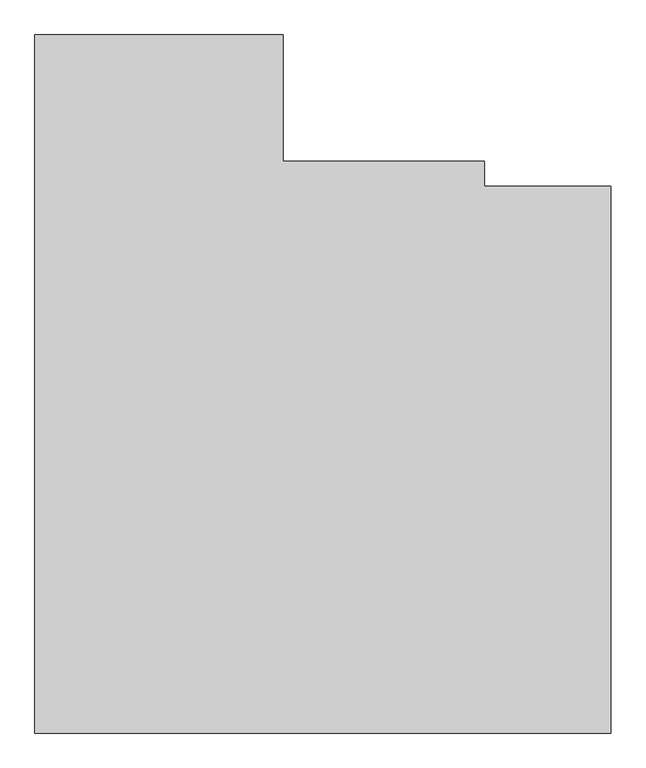
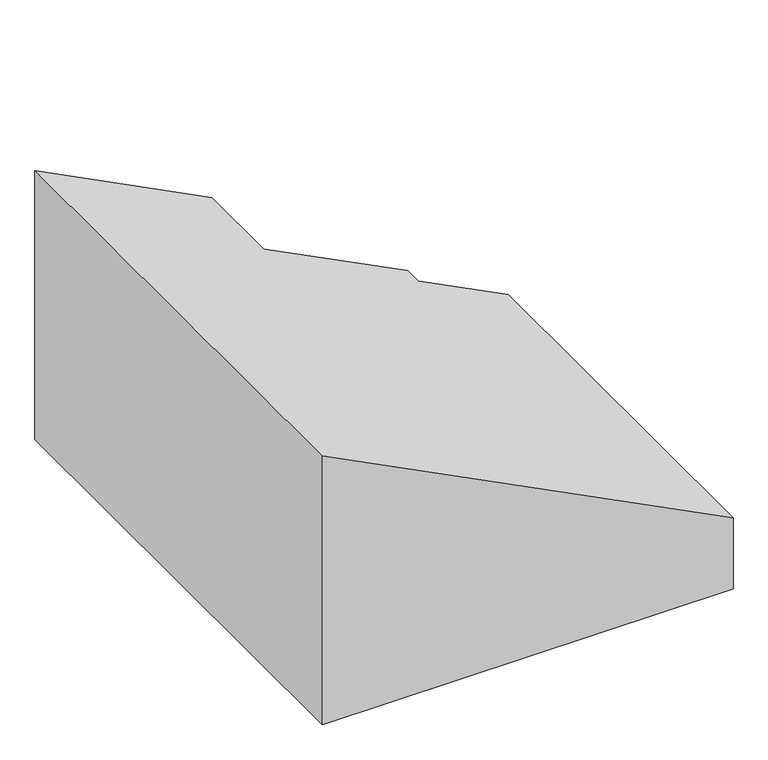
"""IFC4 building model written with IfcOpenShell, lengths in millimetres: proxy geometry, 0_3d_modell."""

import ifcopenshell
import ifcopenshell.guid

model = None  # the IFC model being written
_history = None  # IfcOwnerHistory: only IFC2X3 demands one
_inside = {}  # id of a spatial element -> (the spatial element, [elements in it])
_under = {}  # id of a project, library or spatial element -> (it, [spatial elements below it])
_declared = {}  # id of a project -> (the project, [libraries it declares])
_typed = {}  # id of a type object -> (the type object, [elements of that type])
_made_of = {}  # id of a material, layer set ... -> (it, [elements and type objects made of it])


def new_model(schema):
    """Start an empty IFC model of exactly this schema.

    Asked for "IFC4X3", IfcOpenShell would pick the latest addendum, in which some entities
    have other attributes; the version numbers below select the first issue.
    IFC2X3 requires an IfcOwnerHistory on every rooted entity: one is made here for all.
    """
    global model, _history
    if schema == "IFC4X3":
        model = ifcopenshell.file(schema_version=(4, 3, 0, 0))
    else:
        model = ifcopenshell.file(schema=schema)
    _inside.clear()
    _under.clear()
    _declared.clear()
    _typed.clear()
    _made_of.clear()
    _history = None
    if model.schema == "IFC2X3":
        org = make("IfcOrganization", Name="unknown")
        user = make(
            "IfcPersonAndOrganization",
            ThePerson=make("IfcPerson", FamilyName="unknown"),
            TheOrganization=org,
        )
        app = make(
            "IfcApplication",
            ApplicationDeveloper=org,
            Version="unknown",
            ApplicationFullName="unknown",
            ApplicationIdentifier="unknown",
        )
        _history = make(
            "IfcOwnerHistory",
            OwningUser=user,
            OwningApplication=app,
            ChangeAction="ADDED",
            CreationDate=0,
        )
    return model


def make(cls, **values):
    """One entity of the class cls with the attributes given. An attribute that is None is left unset."""
    return model.create_entity(
        cls, **{name: value for name, value in values.items() if value is not None}
    )


def rooted(cls, **values):
    """An entity with a GlobalId (a new one), such as an element, a storey or a relation."""
    return make(cls, GlobalId=ifcopenshell.guid.new(), OwnerHistory=_history, **values)


def si_unit(unit_type, name, prefix=None):
    """IfcSIUnit, for example si_unit("LENGTHUNIT", "METRE", prefix="MILLI")."""
    return make("IfcSIUnit", UnitType=unit_type, Prefix=prefix, Name=name)


def assignment(units):
    """IfcUnitAssignment: the units of a project."""
    return None if units is None else make("IfcUnitAssignment", Units=units)


def point(xyz):
    """IfcCartesianPoint."""
    return None if xyz is None else make("IfcCartesianPoint", Coordinates=xyz)


def direction(xyz):
    """IfcDirection."""
    return None if xyz is None else make("IfcDirection", DirectionRatios=xyz)


def frame(location, z_axis=None, x_axis=None):
    """IfcAxis2Placement3D, a coordinate frame: its origin and axes. An axis left out is left unset."""
    return make(
        "IfcAxis2Placement3D",
        Location=point(location),
        Axis=direction(z_axis),
        RefDirection=direction(x_axis),
    )


def origin():
    """The frame at (0, 0, 0) with its axes left unset."""
    return frame((0.0, 0.0, 0.0))


def place(relative_to, where):
    """IfcLocalPlacement: puts the frame where relative to a parent placement (None: the world)."""
    return make(
        "IfcLocalPlacement", PlacementRelTo=relative_to, RelativePlacement=where
    )


def context(
    kind, dimensions, precision=None, world=None, true_north=None, identifier=None
):
    """IfcGeometricRepresentationContext, for example the 3D "Model" context."""
    return make(
        "IfcGeometricRepresentationContext",
        ContextIdentifier=identifier,
        ContextType=kind,
        CoordinateSpaceDimension=dimensions,
        Precision=precision,
        WorldCoordinateSystem=world,
        TrueNorth=true_north,
    )


def project(units=None, contexts=None):
    """IfcProject with its units and contexts."""
    return rooted(
        "IfcProject",
        Name="project",
        RepresentationContexts=contexts,
        UnitsInContext=assignment(units),
    )


def spatial(cls, under=None, at=None, **own):
    """A site, building, storey or space (cls), placed at a placement, below another one or the project."""
    s = rooted(cls, ObjectPlacement=at, **own)
    if under is not None:
        _under.setdefault(under.id(), (under, []))[1].append(s)
    return s


def faces_of(points, faces, orient=None, outer=None):
    """IfcFace entities. A face is a list of loops; a loop is a list of indices into points, from 0.

    orient and outer hold one flag for each loop. By default every Orientation is true, the
    first loop of a face is its IfcFaceOuterBound and the others are IfcFaceBound.
    """
    made = []
    for i, loops in enumerate(faces):
        bounds = []
        for j, loop in enumerate(loops):
            is_outer = j == 0 if outer is None else outer[i][j]
            bounds.append(
                make(
                    "IfcFaceOuterBound" if is_outer else "IfcFaceBound",
                    Bound=make("IfcPolyLoop", Polygon=[points[k] for k in loop]),
                    Orientation=True if orient is None else orient[i][j],
                )
            )
        made.append(make("IfcFace", Bounds=bounds))
    return made


def faceted_brep(points, faces, orient=None, outer=None, voids=None):
    """IfcFacetedBrep: a solid bounded by flat faces; with voids (closed shells), ...WithVoids."""
    shared = [point(p) for p in points]
    hull = make("IfcClosedShell", CfsFaces=faces_of(shared, faces, orient, outer))
    if voids is None:
        return make("IfcFacetedBrep", Outer=hull)
    return make(
        "IfcFacetedBrepWithVoids",
        Outer=hull,
        Voids=[
            make(cls, CfsFaces=faces_of(shared, fs, o, b)) for cls, fs, o, b in voids
        ],
    )


def shape(context_of_items, identifier, shape_type, items):
    """IfcShapeRepresentation: the items that make up one representation, for example the "Body"."""
    return make(
        "IfcShapeRepresentation",
        ContextOfItems=context_of_items,
        RepresentationIdentifier=identifier,
        RepresentationType=shape_type,
        Items=items,
    )


def source(mapping_origin, context_of_items, identifier, shape_type, items):
    """IfcRepresentationMap: a shape defined once, which mapped items show again and again."""
    return make(
        "IfcRepresentationMap",
        MappingOrigin=mapping_origin,
        MappedRepresentation=shape(context_of_items, identifier, shape_type, items),
    )


def transform(
    local_origin,
    x_axis=None,
    y_axis=None,
    z_axis=None,
    scale=None,
    scale2=None,
    scale3=None,
    uniform=True,
):
    """IfcCartesianTransformationOperator3D, or its non-uniform kind. x_axis, y_axis, z_axis: its Axis1, 2, 3."""
    if uniform:
        return make(
            "IfcCartesianTransformationOperator3D",
            Axis1=direction(x_axis),
            Axis2=direction(y_axis),
            LocalOrigin=point(local_origin),
            Scale=scale,
            Axis3=direction(z_axis),
        )
    return make(
        "IfcCartesianTransformationOperator3DnonUniform",
        Axis1=direction(x_axis),
        Axis2=direction(y_axis),
        LocalOrigin=point(local_origin),
        Scale=scale,
        Axis3=direction(z_axis),
        Scale2=scale2,
        Scale3=scale3,
    )


def mapped(mapping_source, mapping_target):
    """IfcMappedItem: shows the shape of a source again, moved by a transform."""
    return make(
        "IfcMappedItem", MappingSource=mapping_source, MappingTarget=mapping_target
    )


def made_of(thing, what):
    """Note that an element or type object is made of a material, layer set ...; save() writes the relation."""
    if what is not None:
        _made_of.setdefault(what.id(), (what, []))[1].append(thing)
    return thing


def element(
    cls,
    number,
    at=None,
    inside=None,
    cuts=None,
    type_object=None,
    material=None,
    context=None,
    identifier="Body",
    shape_type=None,
    held_by="IfcProductDefinitionShape",
    body=None,
    shapes=None,
    **own,
):
    """One element of the class cls, such as IfcWall. Its Tag is "e" and its number.

    at: its placement. inside: the storey or other place that contains it. cuts: it is an
    opening in that element (IfcRelVoidsElement). A single representation is given by context,
    identifier, shape_type and body (its items); several are given by shapes. held_by: the class
    of the entity that holds the representations. save() writes the other relations.
    """
    e = rooted(cls, Tag="e%d" % number, ObjectPlacement=at, **own)
    if body is not None:
        shapes = [shape(context, identifier, shape_type, body)]
    if shapes is not None:
        e.Representation = make(held_by, Representations=shapes)
    if inside is not None:
        _inside.setdefault(inside.id(), (inside, []))[1].append(e)
    if cuts is not None:
        rooted(
            "IfcRelVoidsElement", RelatingBuildingElement=cuts, RelatedOpeningElement=e
        )
    if type_object is not None:
        _typed.setdefault(type_object.id(), (type_object, []))[1].append(e)
    return made_of(e, material)


def aggregate(whole, parts):
    """IfcRelAggregates: a whole, such as a stair, and the parts it consists of."""
    return rooted("IfcRelAggregates", RelatingObject=whole, RelatedObjects=parts)


def save(model, path):
    """Write the relations noted so far, then the file.

    IfcRelAggregates (storeys below a building ...), IfcRelContainedInSpatialStructure (elements
    in a storey), IfcRelDefinesByType, IfcRelAssociatesMaterial and IfcRelDeclares: one each for
    every whole, place, type object, material and project.
    """
    for whole, parts in _under.values():
        aggregate(whole, parts)
    for where, things in _inside.values():
        rooted(
            "IfcRelContainedInSpatialStructure",
            RelatedElements=things,
            RelatingStructure=where,
        )
    for kind, things in _typed.values():
        rooted("IfcRelDefinesByType", RelatedObjects=things, RelatingType=kind)
    for what, things in _made_of.values():
        rooted("IfcRelAssociatesMaterial", RelatedObjects=things, RelatingMaterial=what)
    for by, libraries in _declared.values():
        rooted("IfcRelDeclares", RelatingContext=by, RelatedDefinitions=libraries)
    model.write(path)


def generic_models_0269b9af(model_context):
    return source(origin(), model_context, "Body", "Brep", [
        faceted_brep([(4680.0, 4440.2642941, 853.3339073), (3655.0, 4440.2642941, 1375.5974931), (3655.0, 4645.0, 1375.5974931), (2015.3981634, 4645.0, 2211.0163558), (2015.0, 5670.0, 2211.2192302), (0.0, 5670.0, 3237.913011), (0.0, 0.0, 3237.913011), (4680.0, 0.0, 853.3339073), (2015.0, 5670.0, 0.0), (0.0, 5670.0, 0.0), (2015.3981634, 4645.0, 0.0), (3655.0, 4645.0, 0.0), (3655.0, 4440.2642941, 0.0), (4680.0, 4440.2642941, 0.0), (4680.0, 0.0, 0.0), (0.0, 0.0, 0.0)], [[[0, 1, 2, 3, 4, 5, 6, 7]], [[5, 4, 8, 9]], [[4, 3, 10, 8]], [[3, 2, 11, 10]], [[2, 1, 12, 11]], [[1, 0, 13, 12]], [[0, 7, 14, 13]], [[7, 6, 15, 14]], [[9, 15, 6, 5]], [[11, 12, 13, 14, 15, 9, 8, 10]]]),
    ])


if __name__ == "__main__":
    model = new_model("IFC4")
    model_context = context("Model", 3, world=origin())
    ifc_project = project(units=[si_unit("LENGTHUNIT", "METRE", prefix="MILLI")], contexts=[model_context])
    site = spatial("IfcSite", under=ifc_project)
    building = spatial("IfcBuilding", under=site)
    placement = place(None, origin())
    generic_models_shape = generic_models_0269b9af(model_context)
    element("IfcBuildingElementProxy", 1, Name="0_3d_modell", ObjectType="0_3d_modell", at=placement, inside=building, context=model_context, shape_type="MappedRepresentation", body=[
        mapped(generic_models_shape, transform((0.0, 0.0, 0.0), x_axis=(1.0, 0.0, 0.0), y_axis=(0.0, 1.0, 0.0), z_axis=(0.0, 0.0, 1.0))),
    ])
    save(model, "model.ifc")

# Revit data of these elements
# Project information
#   Organization Name = "Organization Name"
#   Organization Description = "Organization Description"
#   Building Name = "Building Name"
#   IfcOrganization = "KURIARCHITEKTEN"
#   IfcApplicationVersion = "2024.1"
#   IfcApplicationName = "Allplan"
#   IfcSite GUID = "3xMs$kp1n46ejeur8tozco"
#   IfcBuilding GUID = "0i8UyhEYT3nv9HLlo1H2X7"
#   IfcProject GUID = "2x1YFttxr4OvBiL8xtaqeA"
#   IfcDecomposes = "BVH Tammik Wohnhaus Waldrain"
#   IfcDecomposesGUID = "2x1YFttxr4OvBiL8xtaqeA"
#   IfcPropertySetList = "\"AllplanAttributes\""
#   BuildingName = "WALDRAIN"
#   SiteName = "BAUANTRAG"
#   IfcProject Name = "BVH Tammik Wohnhaus Waldrain"
#   AllplanAttributes.Land = "IFC - Land"
#   AllplanAttributes.Bundesland = "IFC - Bundesland"
#   AllplanAttributes.Prüfer = "Prüfstatiker"
#   AllplanAttributes.Bauherr = "Jeremy Tammik"
#   AllplanAttributes.Bruttogeschossfläche = "IFC - Bruttogeschossfläche"
#   AllplanAttributes.Projektleiter = "Projektleitername"
#   AllplanAttributes.Architekt = "Architektenname"
#   AllplanAttributes.Statik = "Statiker"
#   AllplanAttributes.Elektro = "Elektroplaner"
#   AllplanAttributes.Heizung = "Heizungsplaner"
#   AllplanAttributes.Sanitär = "Sanitärplaner"
#   AllplanAttributes.Bebaubare Fläche = "IFC - bebaubare Fläche"
#   AllplanAttributes.Maximale Gebäudehöhe = "IFC - Maximale Gebäudehöhe"
#   AllplanAttributes.Bruttogrundstücksfläche = "IFC - Bruttogrundstücksfläche"
#   AllplanAttributes.Normalhöhennull = "IFC - Höhe über NN"
#   AllplanAttributes.Projektvorlage = "IBD 2023"
#   AllplanAttributes.Bauvorhaben = "BVH Waldrain"
#   AllplanAttributes.Bauherr Straße = "Hühnerbergweg 30"
#   AllplanAttributes.Bauherr Plz/Ort = "79539 Lörrach"
#   AllplanAttributes.Architekt Straße = "Architektenstrasse 111"
#   AllplanAttributes.Architekt Plz/Ort = "72108 Architektenort"
#   AllplanAttributes.Bauvorhaben Straße = "Sonnenweg 6"
#   AllplanAttributes.Bauvorhaben Plz/Ort = "79539 Lörrach"
#   AllplanAttributes.Projektnummer = "2023"
#   AllplanAttributes.Architekt Telefonnummer = "07472-93791-0"
#   AllplanAttributes.Architekt Telefaxnummer = "07472/93791-29"
#   AllplanAttributes.Projektbeschreibung = "Projektnamen Ergänzung"
#   AllplanAttributes.Geographische Länge = "IFC - Geografische Länge"
#   AllplanAttributes.Geographische Breite = "IFC - Geografische Breite"
#   AllplanAttributes.Architekt E-Mail = "Architekt@email.de"
#   Original IFC File Name = "Y:\\j\\doc\\house\\huenerberg\\waldrain\\html\\waldrain.github.io\\doc\\biz\\kuri\\2024-06-26\\0_3d_modell.ifc"
#   Original IFC File Size = "6282447"
#   Revit File Last Updated = "638550083480347085"
#   Revit Importer Version = "Importer 25.0.2.419"
#   Import Method = "Hybrid"
#   Project Issue Date = "Issue Date"
#   Project Status = "Project Status"
#   Client Name = "Client Name"
#   Project Address = "Enter address here\nAddress Line 2"
#   Project Name = "Project Name"
#   Project Number = "Project Number"
# Element 1 (IfcBuildingElementProxy, "0_3d_modell")
#   Materials on its faces: "*1"
# Materials
#   "*1": class "Unassigned", colour RGB 175 175 175, transparency 0
